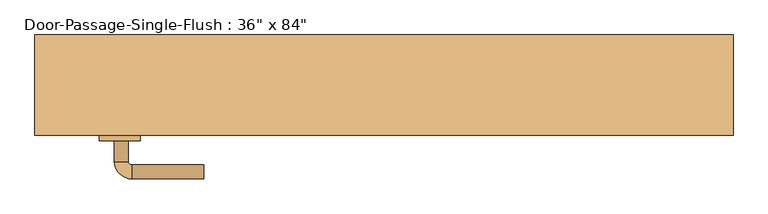
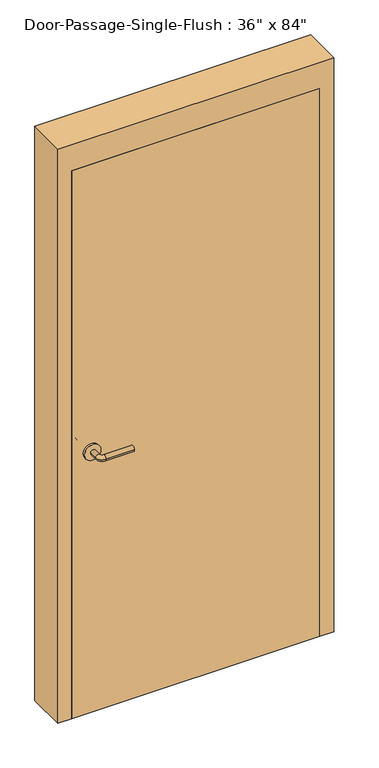
"""IFC4 building model written with IfcOpenShell, lengths in millimetres: door geometry."""

from ifc_helpers import new_model, si_unit, point, frame, frame_2d, origin, origin_with_axes, place, context, project, spatial, polyline, circle_curve, ellipse_curve, trimmed, segment, composite_curve, outline, extrude, faceted_brep, source, transform, mapped, element, save
from ifc_brep_helpers import plane_surface, cylinder_surface, revolved_surface, advanced_brep


def door_01a91e93(model_context):
    return source(origin(), model_context, "Body", "SolidModel", [
        advanced_brep(
        [(-392.190625, -96.775, 1016.0), (-372.190625, -96.775, 1016.0), (-392.190625, -66.775, 1016.0), (-372.190625, -66.775, 1016.0), (-367.190625, -61.775, 1016.0), (-367.190625, -41.775, 1016.0), (-262.190625, -41.775, 1016.0), (-262.190625, -61.775, 1016.0)],
        [
            (0, 1, circle_curve(frame((-382.190625, -96.775, 1016.0), z_axis=(0.0, -1.0, 0.0), x_axis=(1.0, 0.0, 0.0)), 10.0)),
            (1, 0, circle_curve(frame((-382.190625, -96.775, 1016.0), z_axis=(0.0, -1.0, 0.0), x_axis=(1.0, 0.0, 0.0)), 10.0)),
            (0, 2),
            (2, 3, circle_curve(frame((-382.190625, -66.775, 1016.0), z_axis=(0.0, -1.0, 0.0), x_axis=(1.0, 0.0, 0.0)), 10.0)),
            (3, 1),
            (3, 2, circle_curve(frame((-382.190625, -66.775, 1016.0), z_axis=(0.0, -1.0, 0.0), x_axis=(1.0, 0.0, 0.0)), 10.0)),
            (4, 3, circle_curve(frame((-367.190625, -66.775, 1016.0), z_axis=(0.0, 0.0, 1.0), x_axis=(-1.0, 0.0, 0.0)), 5.0)),
            (2, 5, circle_curve(frame((-367.190625, -66.775, 1016.0), z_axis=(0.0, 0.0, -1.0), x_axis=(-1.0, 0.0, 0.0)), 25.0)),
            (5, 4, circle_curve(frame((-367.190625, -51.775, 1016.0), z_axis=(-1.0, 0.0, 0.0), x_axis=(0.0, -1.0, 0.0)), 10.0)),
            (4, 5, circle_curve(frame((-367.190625, -51.775, 1016.0), z_axis=(-1.0, 0.0, 0.0), x_axis=(0.0, -1.0, 0.0)), 10.0)),
            (6, 7, circle_curve(frame((-262.190625, -51.775, 1016.0), z_axis=(1.0, 0.0, 0.0), x_axis=(0.0, -1.0, 0.0)), 10.0)),
            (7, 6, circle_curve(frame((-262.190625, -51.775, 1016.0), z_axis=(1.0, 0.0, 0.0), x_axis=(0.0, -1.0, 0.0)), 10.0)),
            (5, 6),
            (7, 4),
        ],
        [
            plane_surface(frame((-382.190625, -96.775, 1016.0), z_axis=(0.0, -1.0, 0.0), x_axis=(0.0, 0.0, 1.0))),
            cylinder_surface(frame((-382.190625, -96.775, 1016.0), z_axis=(0.0, -1.0, 0.0), x_axis=(1.0, 0.0, 0.0)), 10.0),
            revolved_surface(trimmed(ellipse_curve(frame((-382.190625, -66.775, 1016.0), z_axis=(0.0, -1.0, 0.0), x_axis=(1.0, 0.0, 0.0)), 10.0, 10.0), [point((-392.190625, -66.775, 1016.0))], [point((-372.190625, -66.775, 1016.0))], True, "CARTESIAN"), (-367.190625, -66.775, 1016.0), (0.0, 0.0, -1.0)),
            revolved_surface(trimmed(ellipse_curve(frame((-382.190625, -66.775, 1016.0), z_axis=(0.0, -1.0, 0.0), x_axis=(1.0, 0.0, 0.0)), 10.0, 10.0), [point((-372.190625, -66.775, 1016.0))], [point((-392.190625, -66.775, 1016.0))], True, "CARTESIAN"), (-367.190625, -66.775, 1016.0), (0.0, 0.0, -1.0)),
            plane_surface(frame((-262.190625, -51.775, 1016.0), z_axis=(1.0, 0.0, 0.0), x_axis=(0.0, 0.0, 1.0))),
            cylinder_surface(frame((-367.190625, -51.775, 1016.0), z_axis=(-1.0, 0.0, 0.0), x_axis=(0.0, -1.0, 0.0)), 10.0),
        ],
        [
            (0, [[1, 2]]),
            (1, [[-1, 3, 4, 5]]),
            (1, [[-2, -5, 6, -3]]),
            (2, [[7, -4, 8, 9]]),
            (3, [[-8, -6, -7, 10]]),
            (4, [[11, 12]]),
            (5, [[-9, 13, -12, 14]]),
            (5, [[-10, -14, -11, -13]]),
        ],
    ),
        extrude(outline(composite_curve([segment(trimmed(circle_curve(frame_2d((1016.0, -384.690625)), 30.0), [point((1016.0, -414.690625))], [point((1016.0, -354.690625))], False, "CARTESIAN"), True, "CONTINUOUS"), segment(trimmed(circle_curve(frame_2d((1016.0, -384.690625)), 30.0), [point((1016.0, -354.690625))], [point((1016.0, -414.690625))], False, "CARTESIAN"), True, "CONTINUOUS")], self_intersect=False)), frame((0.0, -104.775, 0.0), z_axis=(0.0, 1.0, 0.0), x_axis=(0.0, 0.0, 1.0)), (0.0, 0.0, 1.0), 8.0),
        advanced_brep(
        [(-392.190625, -157.225, 1016.0), (-372.190625, -157.225, 1016.0), (-372.190625, -187.225, 1016.0), (-392.190625, -187.225, 1016.0), (-367.190625, -192.225, 1016.0), (-367.190625, -212.225, 1016.0), (-262.190625, -212.225, 1016.0), (-262.190625, -192.225, 1016.0)],
        [
            (0, 1, circle_curve(frame((-382.190625, -157.225, 1016.0), z_axis=(0.0, 1.0, 0.0), x_axis=(1.0, 0.0, 0.0)), 10.0)),
            (1, 0, circle_curve(frame((-382.190625, -157.225, 1016.0), z_axis=(0.0, 1.0, 0.0), x_axis=(1.0, 0.0, 0.0)), 10.0)),
            (1, 2),
            (2, 3, circle_curve(frame((-382.190625, -187.225, 1016.0), z_axis=(0.0, 1.0, 0.0), x_axis=(1.0, 0.0, 0.0)), 10.0)),
            (3, 0),
            (3, 2, circle_curve(frame((-382.190625, -187.225, 1016.0), z_axis=(0.0, 1.0, 0.0), x_axis=(1.0, 0.0, 0.0)), 10.0)),
            (4, 5, circle_curve(frame((-367.190625, -202.225, 1016.0), z_axis=(-1.0, 0.0, 0.0), x_axis=(0.0, 1.0, 0.0)), 10.0)),
            (5, 3, circle_curve(frame((-367.190625, -187.225, 1016.0), z_axis=(0.0, 0.0, -1.0), x_axis=(-1.0, 0.0, 0.0)), 25.0)),
            (2, 4, circle_curve(frame((-367.190625, -187.225, 1016.0), z_axis=(0.0, 0.0, 1.0), x_axis=(-1.0, 0.0, 0.0)), 5.0)),
            (5, 4, circle_curve(frame((-367.190625, -202.225, 1016.0), z_axis=(-1.0, 0.0, 0.0), x_axis=(0.0, 1.0, 0.0)), 10.0)),
            (6, 7, circle_curve(frame((-262.190625, -202.225, 1016.0), z_axis=(1.0, 0.0, 0.0), x_axis=(0.0, 1.0, 0.0)), 10.0)),
            (7, 6, circle_curve(frame((-262.190625, -202.225, 1016.0), z_axis=(1.0, 0.0, 0.0), x_axis=(0.0, 1.0, 0.0)), 10.0)),
            (4, 7),
            (6, 5),
        ],
        [
            plane_surface(frame((-382.190625, -157.225, 1016.0), z_axis=(0.0, 1.0, 0.0), x_axis=(0.0, 0.0, 1.0))),
            cylinder_surface(frame((-382.190625, -157.225, 1016.0), z_axis=(0.0, 1.0, 0.0), x_axis=(1.0, 0.0, 0.0)), 10.0),
            revolved_surface(trimmed(ellipse_curve(frame((-382.190625, -187.225, 1016.0), z_axis=(0.0, -1.0, 0.0), x_axis=(1.0, 0.0, 0.0)), 10.0, 10.0), [point((-392.190625, -187.225, 1016.0))], [point((-372.190625, -187.225, 1016.0))], True, "CARTESIAN"), (-367.190625, -187.225, 1016.0), (0.0, 0.0, -1.0)),
            revolved_surface(trimmed(ellipse_curve(frame((-382.190625, -187.225, 1016.0), z_axis=(0.0, -1.0, 0.0), x_axis=(1.0, 0.0, 0.0)), 10.0, 10.0), [point((-372.190625, -187.225, 1016.0))], [point((-392.190625, -187.225, 1016.0))], True, "CARTESIAN"), (-367.190625, -187.225, 1016.0), (0.0, 0.0, -1.0)),
            plane_surface(frame((-262.190625, -202.225, 1016.0), z_axis=(1.0, 0.0, 0.0), x_axis=(0.0, 0.0, 1.0))),
            cylinder_surface(frame((-367.190625, -202.225, 1016.0), z_axis=(-1.0, 0.0, 0.0), x_axis=(0.0, 1.0, 0.0)), 10.0),
        ],
        [
            (0, [[1, 2]]),
            (1, [[3, 4, 5, -2]]),
            (1, [[-5, 6, -3, -1]]),
            (2, [[7, 8, -4, 9]]),
            (3, [[10, -9, -6, -8]]),
            (4, [[11, 12]]),
            (5, [[13, -11, 14, -7]]),
            (5, [[-14, -12, -13, -10]]),
        ],
    ),
        extrude(outline(composite_curve([segment(trimmed(circle_curve(frame_2d((1016.0, -384.690625)), 30.0), [point((1016.0, -414.690625))], [point((1016.0, -354.690625))], False, "CARTESIAN"), True, "CONTINUOUS"), segment(trimmed(circle_curve(frame_2d((1016.0, -384.690625)), 30.0), [point((1016.0, -354.690625))], [point((1016.0, -414.690625))], False, "CARTESIAN"), True, "CONTINUOUS")], self_intersect=False)), frame((0.0, -157.225, 0.0), z_axis=(0.0, 1.0, 0.0), x_axis=(0.0, 0.0, 1.0)), (0.0, 0.0, 1.0), 8.0),
        faceted_brep([(457.2, -100.0125, 0.0), (441.325, -100.0125, 0.0), (441.325, -52.3875, 0.0), (457.2, -52.3875, 0.0), (457.2, -3.175, 0.0), (508.0, -3.175, 0.0), (508.0, -149.225, 0.0), (457.2, -149.225, 0.0), (457.2, -149.225, 2133.6), (457.2, -100.0125, 2133.6), (508.0, -149.225, 2235.2), (-508.0, -149.225, 2235.2), (-508.0, -149.225, 0.0), (-457.2, -149.225, 0.0), (-457.2, -149.225, 2133.6), (508.0, -3.175, 2235.2), (457.2, -3.175, 2133.6), (-457.2, -3.175, 2133.6), (-457.2, -3.175, 0.0), (-508.0, -3.175, 0.0), (-508.0, -3.175, 2235.2), (457.2, -52.3875, 2133.6), (441.325, -52.3875, 2117.725), (-441.325, -52.3875, 2117.725), (-441.325, -52.3875, 0.0), (-457.2, -52.3875, 0.0), (-457.2, -52.3875, 2133.6), (441.325, -100.0125, 2117.725), (-457.2, -100.0125, 2133.6), (-457.2, -100.0125, 0.0), (-441.325, -100.0125, 0.0), (-441.325, -100.0125, 2117.725)], [[[0, 1, 2, 3, 4, 5, 6, 7]], [[7, 8, 9, 0]], [[6, 10, 11, 12, 13, 14, 8, 7]], [[5, 15, 10, 6]], [[4, 16, 17, 18, 19, 20, 15, 5]], [[3, 21, 16, 4]], [[2, 22, 23, 24, 25, 26, 21, 3]], [[1, 27, 22, 2]], [[0, 9, 28, 29, 30, 31, 27, 1]], [[8, 14, 28, 9]], [[16, 21, 26, 17]], [[22, 27, 31, 23]], [[12, 19, 18, 25, 24, 30, 29, 13]], [[13, 29, 28, 14]], [[11, 20, 19, 12]], [[17, 26, 25, 18]], [[23, 31, 30, 24]], [[15, 20, 11, 10]]]),
        extrude(outline(polyline([(457.2, -104.775), (457.2, -149.225), (-457.2, -149.225), (-457.2, -104.775), (457.2, -104.775)])), origin_with_axes(), (0.0, 0.0, 1.0), 2133.6),
    ])


if __name__ == "__main__":
    model = new_model("IFC4")
    model_context = context("Model", 3, world=origin())
    ifc_project = project(units=[si_unit("LENGTHUNIT", "METRE", prefix="MILLI")], contexts=[model_context])
    site = spatial("IfcSite", under=ifc_project)
    building = spatial("IfcBuilding", under=site)
    placement = place(None, origin())
    door_shape = door_01a91e93(model_context)
    element("IfcDoor", 1, ObjectType="Door-Passage-Single-Flush : 36\" x 84\"", at=placement, inside=building, context=model_context, shape_type="MappedRepresentation", body=[
        mapped(door_shape, transform((0.0, 0.0, 0.0), x_axis=(1.0, 0.0, 0.0), y_axis=(0.0, 1.0, 0.0), z_axis=(0.0, 0.0, 1.0))),
    ])
    save(model, "model.ifc")

# Revit data of these elements
# Type "Door-Passage-Single-Flush : 36\" x 84\""
#   Type Mark = "1"
#   Assembly Code = "B2030200"
#   Analytic Construction = "Wooden"
#   Thickness = 0' - 1 3/4"
#   Thermal Resistance (R) = 2.5876 (h·ft²·°F)/BTU
#   Swing Angle [instance default] = 90.00°
#   Strike Height = 3' - 4"
#   Rough Width [instance default] = 3' - 4"
#   Rough Height [instance default] = 7' - 4"
#   MF Opening Height [instance default] = 0' - 4"
#   MF Opening Width [instance default] = 0' - 4"
#   Inset Calculate [instance default] = 0' - 4"
#   Masonry Inset [instance default] = 0' - 1"
#   Height = 7' - 0"
#   Width = 3' - 0"
#   Heat Transfer Coefficient (U) = 0.3865 BTU/(h·ft²·°F)
#   Masonry Frame Depth = 0' - 5 3/4"
#   Define Thermal Properties by = 1
#   Masonry Frame [instance default] = yes
#   Function = 1
#   Dry Wall Frame [instance default] = no
#   Panel Material = Wood - Birch
#   Frame Material = Metal - Paint Finish - Grey
#   Door Handle Material = Aluminum
#   Visual Light Transmittance = 0
#   Solar Heat Gain Coefficient = 0
#   Wall Closure = (empty or 0)
# Element 1 (IfcDoor, "Door-Passage-Single-Flush : 36\" x 84\"")
#   Materials on its faces: "Aluminum", "Metal - Paint Finish - Grey", "Wood - Birch"
# Materials
#   "Wood - Birch": class "Wood", colour RGB 166 116 52, transparency 0, Cost = 0
#   "Metal - Paint Finish - Grey": class "Paint", colour RGB 104 104 104, transparency 0, Cost = 0
#   "Aluminum": class "Metal", colour RGB 247 247 247, transparency 0, Description = "Aluminum 6061", Cost = 0
